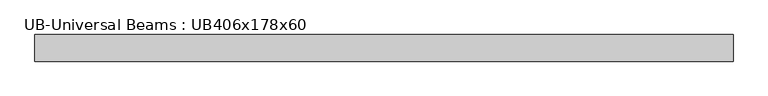
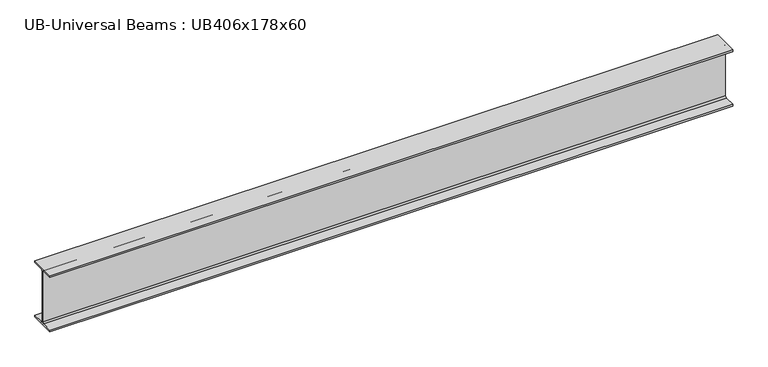
"""IFC4 building model written with IfcOpenShell, lengths in millimetres: beam geometry, UB-Universal Beams : UB406x178x60."""

from ifc_helpers import new_model, si_unit, point, frame, frame_2d, origin, place, context, project, spatial, polyline, circle_curve, trimmed, segment, composite_curve, outline, extrude, source, transform, mapped, element, save


def ub_universal_beams_ub406x178x60_873acc54(model_context):
    return source(origin(), model_context, "Body", "SweptSolid", [
        extrude(outline(composite_curve([segment(polyline([(88.95, -190.4), (88.95, -203.2), (-88.95, -203.2), (-88.95, -190.4), (-14.15, -190.4)]), True, "CONTINUOUS"), segment(trimmed(circle_curve(frame_2d((-14.15, -180.2)), 10.2), [point((-14.15, -190.4))], [point((-3.95, -180.2))], True, "CARTESIAN"), True, "CONTINUOUS"), segment(polyline([(-3.95, -180.2), (-3.95, 180.2)]), True, "CONTINUOUS"), segment(trimmed(circle_curve(frame_2d((-14.15, 180.2)), 10.2), [point((-3.95, 180.2))], [point((-14.15, 190.4))], True, "CARTESIAN"), True, "CONTINUOUS"), segment(polyline([(-14.15, 190.4), (-88.95, 190.4), (-88.95, 203.2), (88.95, 203.2), (88.95, 190.4), (14.15, 190.4)]), True, "CONTINUOUS"), segment(trimmed(circle_curve(frame_2d((14.15, 180.2)), 10.2), [point((14.15, 190.4))], [point((3.95, 180.2))], True, "CARTESIAN"), True, "CONTINUOUS"), segment(polyline([(3.95, 180.2), (3.95, -180.2)]), True, "CONTINUOUS"), segment(trimmed(circle_curve(frame_2d((14.15, -180.2)), 10.2), [point((3.95, -180.2))], [point((14.15, -190.4))], True, "CARTESIAN"), True, "CONTINUOUS"), segment(polyline([(14.15, -190.4), (88.95, -190.4)]), True, "CONTINUOUS")], self_intersect=False)), frame((-2333.3, 0.0, 0.0), z_axis=(1.0, 0.0, 0.0), x_axis=(0.0, 1.0, 0.0)), (0.0, 0.0, 1.0), 4666.6),
    ])


if __name__ == "__main__":
    model = new_model("IFC4")
    model_context = context("Model", 3, world=origin())
    ifc_project = project(units=[si_unit("LENGTHUNIT", "METRE", prefix="MILLI")], contexts=[model_context])
    site = spatial("IfcSite", under=ifc_project)
    building = spatial("IfcBuilding", under=site)
    placement = place(None, origin())
    ub_universal_beams_ub406x178x60_shape = ub_universal_beams_ub406x178x60_873acc54(model_context)
    element("IfcBeam", 1, ObjectType="UB-Universal Beams : UB406x178x60", at=placement, inside=building, context=model_context, shape_type="MappedRepresentation", body=[
        mapped(ub_universal_beams_ub406x178x60_shape, transform((0.0, 0.0, 0.0), x_axis=(1.0, 0.0, 0.0), y_axis=(0.0, 1.0, 0.0), z_axis=(0.0, 0.0, 1.0))),
    ])
    save(model, "model.ifc")

# Revit data of these elements
# Type "UB-Universal Beams : UB406x178x60"
#   Section Name Key = "UB406X178X60"
#   Width = 17.79 cm
#   Web Thickness = 0.79 cm
#   Web Fillet = 1.02 cm
#   Warping Constant = 466000.0 cm⁶
#   Torsional Moment of Inertia = 33.30 cm⁴
#   Section Area = 76.5 cm²
#   Plastic Modulus weak axis = 209.0 cm³
#   Plastic Modulus strong axis = 1200.0 cm³
#   Nominal Weight = 60.0998 kgf/m
#   Moment of Inertia weak axis = 1203.00 cm⁴
#   Moment of Inertia strong axis = 21596.00 cm⁴
#   Height = 40.64 cm
#   Flange Thickness = 1.28 cm
#   Elastic Modulus weak axis = 135.0 cm³
#   Elastic Modulus strong axis = 1063.0 cm³
#   Centroid Vertical = 20.32 cm
#   Centroid Horizontal = 8.895 cm
#   Bolt Spacing = 9.0 cm
#   Length [instance default] = 1500 mm
#   Structural Material [instance default] = Metal - Steel 43-275
#   Type Comments = ""
#   Assembly Code = ""
# Element 1 (IfcBeam, "UB-Universal Beams : UB406x178x60")
#   Materials on its faces: "Metal - Steel 43-275"
# Materials
#   "Metal - Steel 43-275": class "Metal", colour RGB 247 247 247, transparency 0, Cost = 0
